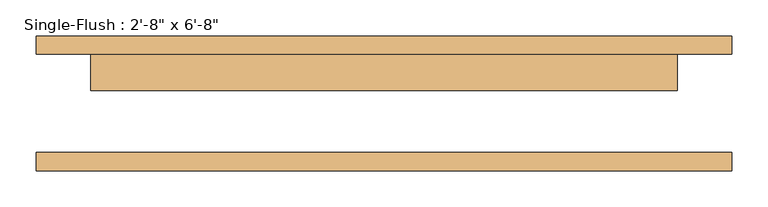
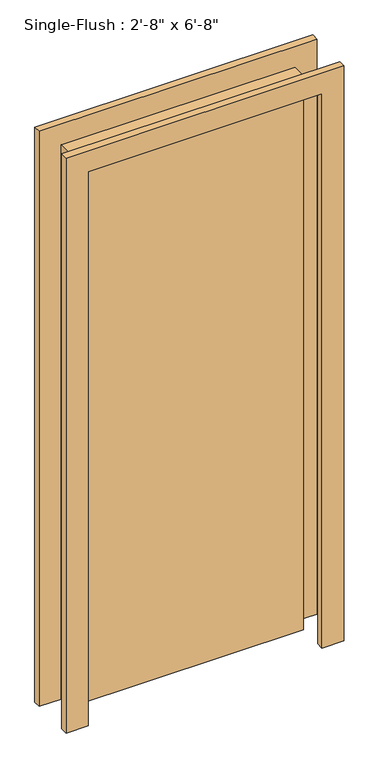
"""IFC4 building model written with IfcOpenShell, lengths in millimetres: door geometry."""

from ifc_helpers import new_model, si_unit, frame, origin, origin_with_axes, place, context, project, spatial, polyline, outline, extrude, source, transform, mapped, element, save


def door_2fa8c1c4(model_context):
    return source(origin(), model_context, "Body", "SweptSolid", [
        extrude(outline(polyline([(2108.2, -482.6), (0.0, -482.6), (0.0, -406.4), (2032.0, -406.4), (2032.0, 406.4), (0.0, 406.4), (0.0, 482.6), (2108.2, 482.6), (2108.2, -482.6)])), frame((0.0, 68.2625, 0.0), z_axis=(0.0, 1.0, 0.0), x_axis=(0.0, 0.0, 1.0)), (0.0, 0.0, 1.0), 25.4),
        extrude(outline(polyline([(2108.2, 482.6), (2108.2, -482.6), (0.0, -482.6), (0.0, -406.4), (2032.0, -406.4), (2032.0, 406.4), (0.0, 406.4), (0.0, 482.6), (2108.2, 482.6)])), frame((0.0, -93.6625, 0.0), z_axis=(0.0, 1.0, 0.0), x_axis=(0.0, 0.0, 1.0)), (0.0, 0.0, 1.0), 25.4),
        extrude(outline(polyline([(406.4, 17.4625), (-406.4, 17.4625), (-406.4, 68.2625), (406.4, 68.2625), (406.4, 17.4625)])), origin_with_axes(), (0.0, 0.0, 1.0), 2032.0),
    ])


if __name__ == "__main__":
    model = new_model("IFC4")
    model_context = context("Model", 3, world=origin())
    ifc_project = project(units=[si_unit("LENGTHUNIT", "METRE", prefix="MILLI")], contexts=[model_context])
    site = spatial("IfcSite", under=ifc_project)
    building = spatial("IfcBuilding", under=site)
    placement = place(None, origin())
    door_shape = door_2fa8c1c4(model_context)
    element("IfcDoor", 1, ObjectType="Single-Flush : 2'-8\" x 6'-8\"", at=placement, inside=building, context=model_context, shape_type="MappedRepresentation", body=[
        mapped(door_shape, transform((0.0, 0.0, 0.0), x_axis=(1.0, 0.0, 0.0), y_axis=(0.0, 1.0, 0.0), z_axis=(0.0, 0.0, 1.0))),
    ])
    save(model, "model.ifc")

# Revit data of these elements
# Type "Single-Flush : 2'-8\" x 6'-8\""
#   Type Mark = "11"
#   Construction Type Id = "MDOOR"
#   Assembly Code = "C1020"
#   Analytic Construction = "Metal"
#   Thickness = 0' - 2"
#   Heat Transfer Coefficient (U) = 3.7021 W/(m²·K)
#   Height = 6' - 8"
#   Trim Projection Ext = 0' - 1"
#   Trim Projection Int = 0' - 1"
#   Trim Width = 0' - 3"
#   Width = 2' - 8"
#   Door Material = Door - Panel
#   Frame Material = Door - Frame
#   Visual Light Transmittance = 0
#   Solar Heat Gain Coefficient = 0
#   Function = (empty or 0)
#   Wall Closure = (empty or 0)
# Element 1 (IfcDoor, "Single-Flush : 2'-8\" x 6'-8\"")
#   Materials on its faces: "Door - Frame", "Door - Panel"
# Materials
#   "Door - Panel": class "Wood", colour RGB 210 159 95, transparency 0, Cost = 0
#   "Door - Frame": class "Miscellaneous", colour RGB 118 70 51, transparency 0, Cost = 0
